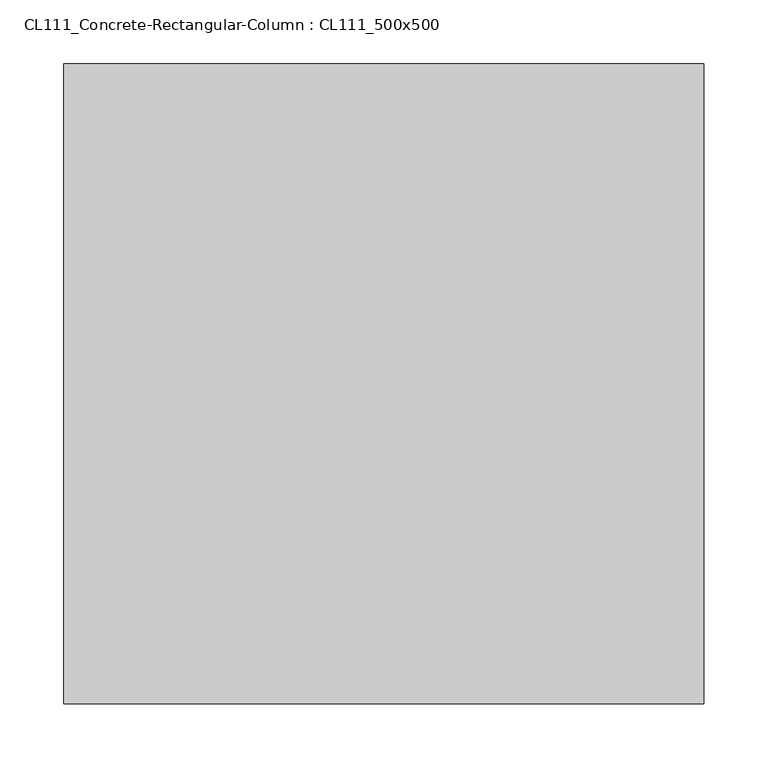
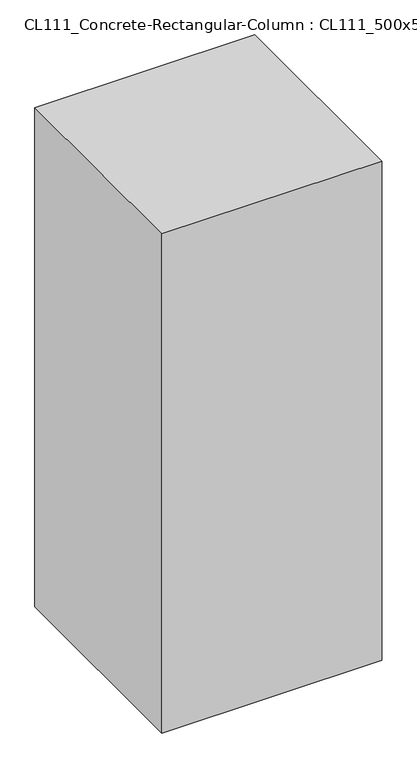
"""IFC4 building model written with IfcOpenShell, lengths in millimetres: column geometry, CL111_Concrete-Rectangular-Column : CL111_500x500."""

from ifc_helpers import new_model, si_unit, frame, origin, place, context, project, spatial, polyline, outline, extrude, source, transform, mapped, element, save


def cl111_concrete_rectangular_column_cl111_500x500_13a722a7(model_context):
    return source(origin(), model_context, "Body", "SweptSolid", [
        extrude(outline(polyline([(250.0, 250.0), (250.0, -250.0), (-250.0, -250.0), (-250.0, 250.0), (250.0, 250.0)])), frame((0.0, 0.0, -1200.0), z_axis=(0.0, 0.0, 1.0), x_axis=(1.0, 0.0, 0.0)), (0.0, 0.0, 1.0), 1200.0),
    ])


if __name__ == "__main__":
    model = new_model("IFC4")
    model_context = context("Model", 3, world=origin())
    ifc_project = project(units=[si_unit("LENGTHUNIT", "METRE", prefix="MILLI")], contexts=[model_context])
    site = spatial("IfcSite", under=ifc_project)
    building = spatial("IfcBuilding", under=site)
    placement = place(None, origin())
    cl111_concrete_rectangular_column_cl111_500x500_shape = cl111_concrete_rectangular_column_cl111_500x500_13a722a7(model_context)
    element("IfcColumn", 1, ObjectType="CL111_Concrete-Rectangular-Column : CL111_500x500", at=placement, inside=building, context=model_context, shape_type="MappedRepresentation", body=[
        mapped(cl111_concrete_rectangular_column_cl111_500x500_shape, transform((0.0, 0.0, 0.0), x_axis=(1.0, 0.0, 0.0), y_axis=(0.0, 1.0, 0.0), z_axis=(0.0, 0.0, 1.0))),
    ])
    save(model, "model.ifc")

# Revit data of these elements
# Type "CL111_Concrete-Rectangular-Column : CL111_500x500"
#   Assembly Code = "B10"
#   b = 500 mm
#   h = 500 mm
#   Structural Material [instance default] = Concrete, Cast-in-Place gray
# Element 1 (IfcColumn, "CL111_Concrete-Rectangular-Column : CL111_500x500")
#   Materials on its faces: "Concrete, Cast-in-Place gray"
# Materials
#   "Concrete, Cast-in-Place gray": class "Concrete", colour RGB 192 192 192, transparency 0, Description = "Cast-in-place concrete", Cost = 0
